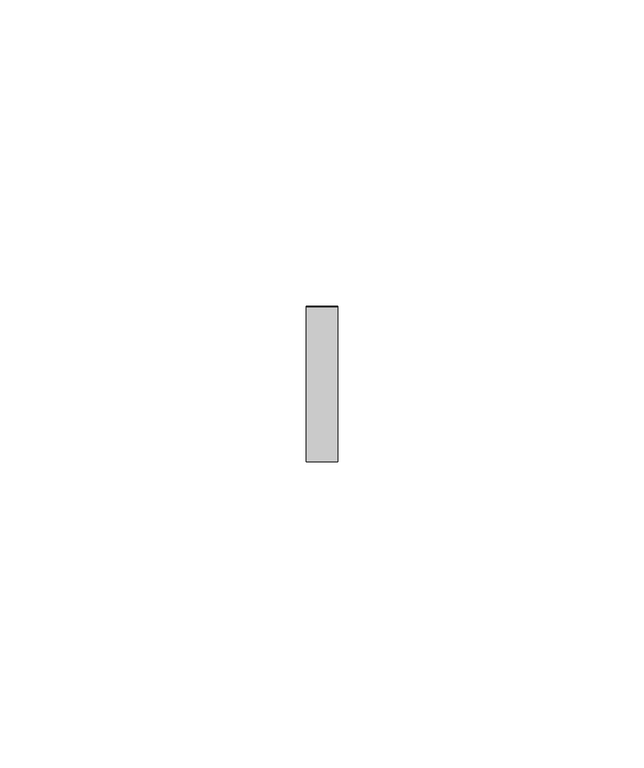
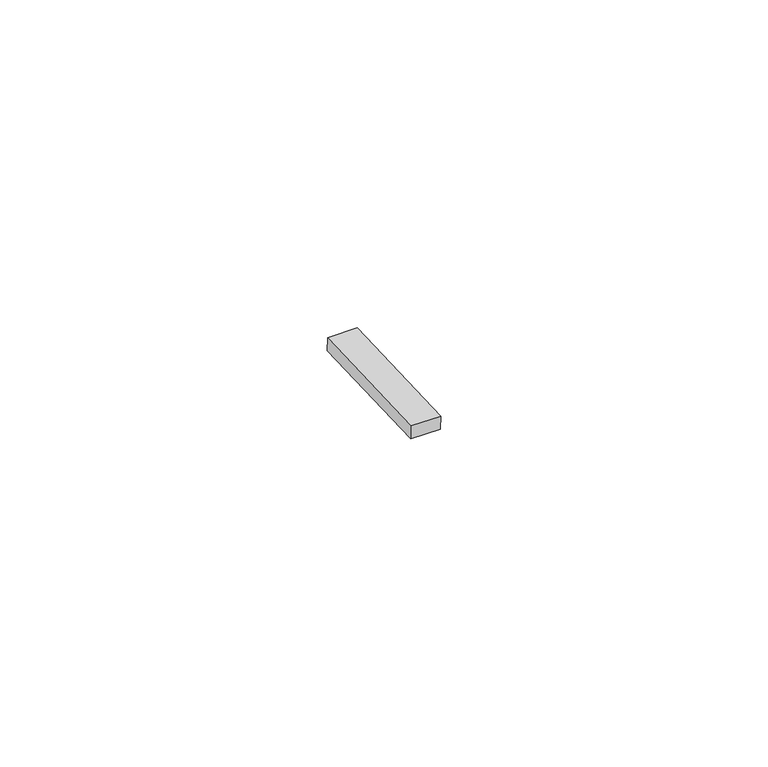
"""IFC4 building model written with IfcOpenShell, lengths in millimetres: proxy geometry, Inner panel:Inner panel:1:Inner panel:1 : Inner panel:Inner panel:300324:2:Inner panel:1:Inner panel:1 : Inner panel:Inner panel:300324:2 : Inner panel:Inner panel:1:Inner panel:1 : Inner panel:Inner panel:300324:300043:136 : Inner panel:Inner panel:1:Inner panel:1 : Inner panel:Inner panel:300324:2:Inner panel:1:Inner panel:1 : Inner panel:Inner panel:300324:2 : Inner panel:Inner panel:1:Inner panel:1 : Inner panel:Inner panel:300324:300043:308120."""

from ifc_helpers import new_model, si_unit, frame, origin, place, context, project, spatial, polyline, outline, extrude, source, transform, mapped, element, save


def generic_models_e81f58e9(model_context):
    return source(origin(), model_context, "Body", "SweptSolid", [
        extrude(outline(polyline([(0.0, -25.3999999), (0.0, 0.0), (5.2138089, 0.0), (5.2138089, -25.3999999), (0.0, -25.3999999)])), frame((592310.995117, -568123.7593241, 8806.3160403), z_axis=(0.0, -0.041630544712223896, 0.9991330730923502), x_axis=(-1.0, 0.0, 0.0)), (0.0, 0.0, 1.0), 2.4763745),
    ])


if __name__ == "__main__":
    model = new_model("IFC4")
    model_context = context("Model", 3, world=origin())
    ifc_project = project(units=[si_unit("LENGTHUNIT", "METRE", prefix="MILLI")], contexts=[model_context])
    site = spatial("IfcSite", under=ifc_project)
    building = spatial("IfcBuilding", under=site)
    placement = place(None, origin())
    generic_models_shape = generic_models_e81f58e9(model_context)
    element("IfcBuildingElementProxy", 1, Name="Inner panel:Inner panel:1:Inner panel:1 : Inner panel:Inner panel:300324:2:Inner panel:1:Inner panel:1 : Inner panel:Inner panel:300324:2 : Inner panel:Inner panel:1:Inner panel:1 : Inner panel:Inner panel:300324:300043:136 : Inner panel:Inner panel:1:Inner panel:1 : Inner panel:Inner panel:300324:2:Inner panel:1:Inner panel:1 : Inner panel:Inner panel:300324:2 : Inner panel:Inner panel:1:Inner panel:1 : Inner panel:Inner panel:300324:300043:308120", ObjectType="Inner panel:Inner panel:1:Inner panel:1 : Inner panel:Inner panel:300324:2:Inner panel:1:Inner panel:1 : Inner panel:Inner panel:300324:2 : Inner panel:Inner panel:1:Inner panel:1 : Inner panel:Inner panel:300324:300043:136 : Inner panel:Inner panel:1:Inner panel:1 : Inner panel:Inner panel:300324:2:Inner panel:1:Inner panel:1 : Inner panel:Inner panel:300324:2 : Inner panel:Inner panel:1:Inner panel:1 : Inner panel:Inner panel:300324:300043:308120", at=placement, inside=building, context=model_context, shape_type="MappedRepresentation", body=[
        mapped(generic_models_shape, transform((0.0, 0.0, 0.0), x_axis=(1.0, 0.0, 0.0), y_axis=(0.0, 1.0, 0.0), z_axis=(0.0, 0.0, 1.0))),
    ])
    save(model, "model.ifc")

# Revit data of these elements
# Type "Inner panel:Inner panel:1:Inner panel:1 : Inner panel:Inner panel:300324:2:Inner panel:1:Inner panel:1 : Inner panel:Inner panel:300324:2 : Inner panel:Inner panel:1:Inner panel:1 : Inner panel:Inner panel:300324:300043:136 : Inner panel:Inner panel:1:Inner panel:1 : Inner panel:Inner panel:300324:2:Inner panel:1:Inner panel:1 : Inner panel:Inner panel:300324:2 : Inner panel:Inner panel:1:Inner panel:1 : Inner panel:Inner panel:300324:300043:308120"
#   NameOverride = "Inner panel:Inner panel:1:Inner panel:1 : Inner panel:Inner panel:300324:2:Inner panel:1:Inner panel:1 : Inner panel:Inner panel:300324:2 : Inner panel:Inner panel:1:Inner panel:1 : Inner panel:Inner panel:300324:300043:308120"
#   ObjectTypeOverride = "Inner panel:1:Inner panel:1 : Inner panel:Inner panel:300324:2 : Inner panel:Inner panel:1:Inner panel:1 : Inner panel:Inner panel:300324:300043"
#   Reference = "Inner panel"
#   Tag = "308120"
# Element 1 (IfcBuildingElementProxy, "Inner panel:Inner panel:1:Inner panel:1 : Inner panel:Inner panel:300324:2:Inner panel:1:Inner panel:1 : Inner panel:Inner panel:300324:2 : Inner panel:Inner panel:1:Inner panel:1 : Inner panel:Inner panel:300324:300043:136 : Inner panel:Inner panel:1:Inner panel:1 : Inner panel:Inner panel:300324:2:Inner panel:1:Inner panel:1 : Inner panel:Inner panel:300324:2 : Inner panel:Inner panel:1:Inner panel:1 : Inner panel:Inner panel:300324:300043:308120")
#   Materials on its faces: "AT CLIP - 1\" WIDE NON ABSORBENT, WEATHER-RESISTANT NEOPRENE/EPDM/SBR FOAM"
# Materials
#   "AT CLIP - 1\" WIDE NON ABSORBENT, WEATHER-RESISTANT NEOPRENE/EPDM/SBR FOAM": class "Generic", colour RGB 85 85 85, transparency 0, Cost = 0
